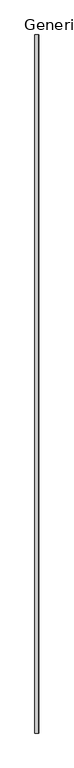
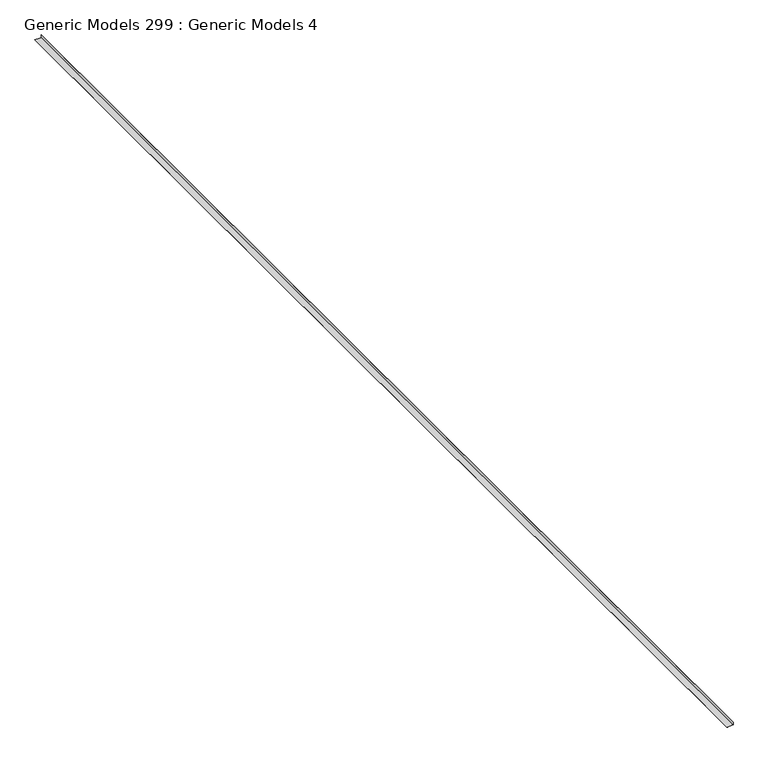
"""IFC4 building model written with IfcOpenShell, lengths in millimetres: proxy geometry, Generic Models 299 : Generic Models 4."""

from ifc_helpers import new_model, si_unit, frame, origin, place, context, project, spatial, polyline, outline, extrude, source, transform, mapped, element, save


def generic_models_299_generic_models_4_73852820(model_context):
    return source(origin(), model_context, "Body", "SweptSolid", [
        extrude(outline(polyline([(124907.5564353, 87413.1799276), (124907.5564353, 87313.815657), (124906.7626853, 87313.815657), (124906.7626853, 87413.9736776), (124953.1020331, 87413.9736776), (124953.1020331, 87413.1799276), (124907.5564353, 87413.1799276)])), frame((0.0, 16287.5029335, 0.0), z_axis=(0.0, 1.0, 0.0), x_axis=(0.0, 0.0, 1.0)), (0.0, 0.0, 1.0), 18643.6),
    ])


if __name__ == "__main__":
    model = new_model("IFC4")
    model_context = context("Model", 3, world=origin())
    ifc_project = project(units=[si_unit("LENGTHUNIT", "METRE", prefix="MILLI")], contexts=[model_context])
    site = spatial("IfcSite", under=ifc_project)
    building = spatial("IfcBuilding", under=site)
    placement = place(None, origin())
    generic_models_299_generic_models_4_shape = generic_models_299_generic_models_4_73852820(model_context)
    element("IfcBuildingElementProxy", 1, Name="Generic Models 299 : Generic Models 4", ObjectType="Generic Models 299 : Generic Models 4", at=placement, inside=building, context=model_context, shape_type="MappedRepresentation", body=[
        mapped(generic_models_299_generic_models_4_shape, transform((0.0, 0.0, 0.0), x_axis=(1.0, 0.0, 0.0), y_axis=(0.0, 1.0, 0.0), z_axis=(0.0, 0.0, 1.0))),
    ])
    save(model, "model.ifc")

# Revit data of these elements
# Element 1 (IfcBuildingElementProxy, "Generic Models 299 : Generic Models 4")
#   Materials on its faces: "_SELF ADHERED MEMBRANE W/ END DAMS WHERE POSSIBLE"
# Materials
#   "_SELF ADHERED MEMBRANE W/ END DAMS WHERE POSSIBLE": class "Generic", colour RGB 253 192 103, transparency 0, Cost = 0
